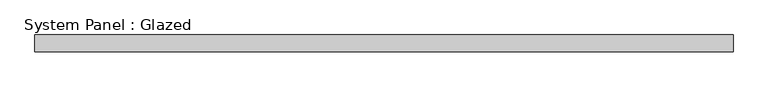
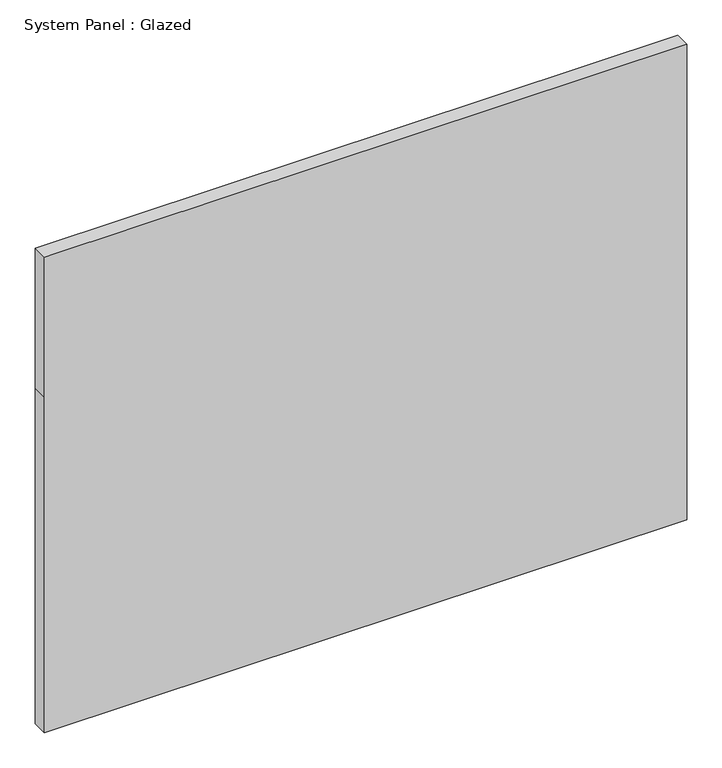
"""IFC4 building model written with IfcOpenShell, lengths in millimetres: plate geometry, System Panel : Glazed."""

from ifc_helpers import new_model, si_unit, frame, origin, place, context, project, spatial, polyline, outline, extrude, source, transform, mapped, element, save


def system_panel_glazed_0ad46d88(model_context):
    return source(origin(), model_context, "Body", "SweptSolid", [
        extrude(outline(polyline([(0.0, -523.0731356), (0.0, 523.0731356), (577.85, 523.0731356), (819.15, 523.0731356), (819.15, -523.0731356), (577.85, -523.0731356), (0.0, -523.0731356)])), frame((0.0, -44.45, 0.0), z_axis=(0.0, 1.0, 0.0), x_axis=(0.0, 0.0, 1.0)), (0.0, 0.0, 1.0), 25.4),
    ])


if __name__ == "__main__":
    model = new_model("IFC4")
    model_context = context("Model", 3, world=origin())
    ifc_project = project(units=[si_unit("LENGTHUNIT", "METRE", prefix="MILLI")], contexts=[model_context])
    site = spatial("IfcSite", under=ifc_project)
    building = spatial("IfcBuilding", under=site)
    placement = place(None, origin())
    system_panel_glazed_shape = system_panel_glazed_0ad46d88(model_context)
    element("IfcPlate", 1, ObjectType="System Panel : Glazed", at=placement, inside=building, context=model_context, shape_type="MappedRepresentation", body=[
        mapped(system_panel_glazed_shape, transform((0.0, 0.0, 0.0), x_axis=(1.0, 0.0, 0.0), y_axis=(0.0, 1.0, 0.0), z_axis=(0.0, 0.0, 1.0))),
    ])
    save(model, "model.ifc")

# Revit data of these elements
# Element 1 (IfcPlate, "System Panel : Glazed")
#   Materials on its faces: "Glass"
# Materials
#   "Glass": class "Unassigned", colour RGB 147 173 200, transparency 0.7, Cost = 0
